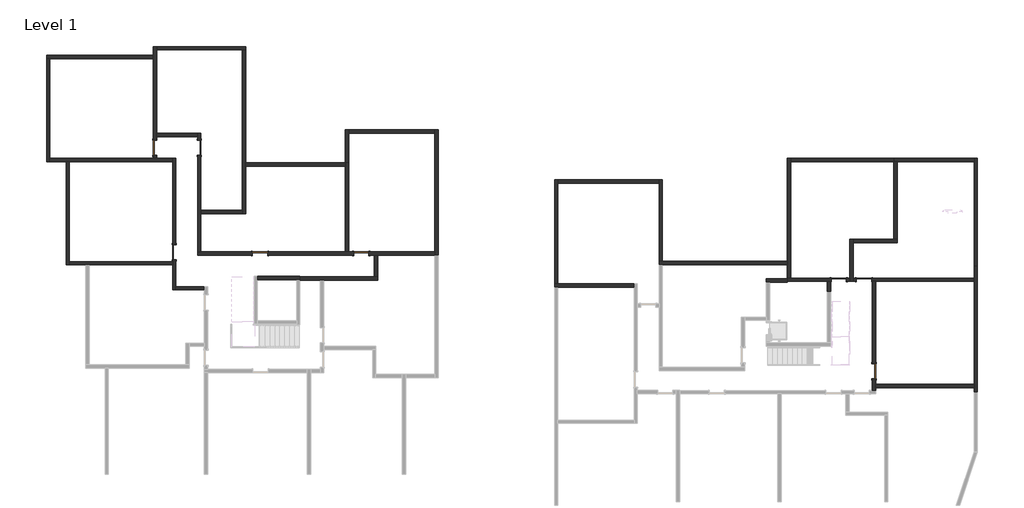
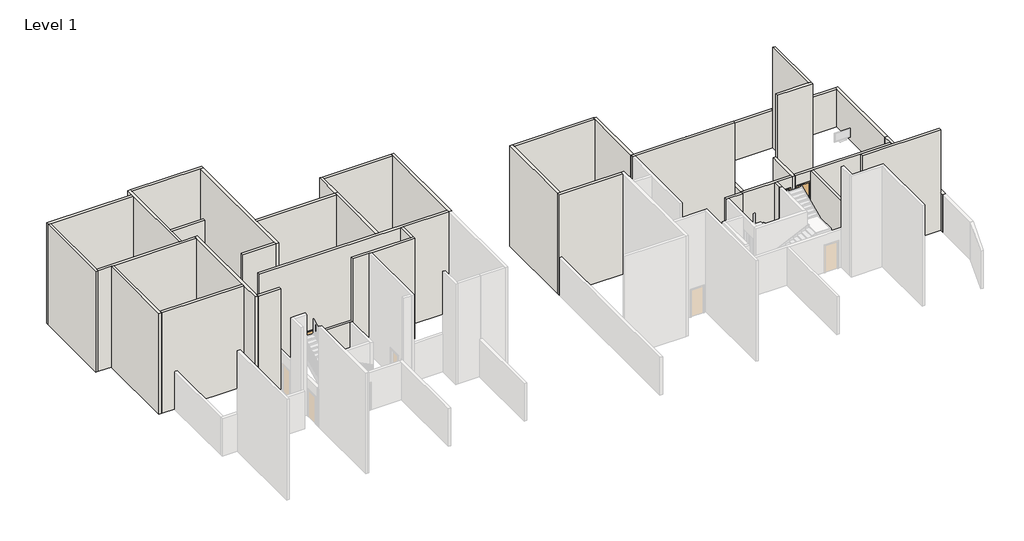
# One storey, part 2 of 3: 41 walls, 8 doors.
"""IFC4 building model written with IfcOpenShell, lengths in millimetres."""

import ifcopenshell
import ifcopenshell.guid

model = None  # the IFC model being written
_history = None  # IfcOwnerHistory: only IFC2X3 demands one
_inside = {}  # id of a spatial element -> (the spatial element, [elements in it])
_under = {}  # id of a project, library or spatial element -> (it, [spatial elements below it])
_declared = {}  # id of a project -> (the project, [libraries it declares])
_typed = {}  # id of a type object -> (the type object, [elements of that type])
_made_of = {}  # id of a material, layer set ... -> (it, [elements and type objects made of it])


def new_model(schema):
    """Start an empty IFC model of exactly this schema.

    Asked for "IFC4X3", IfcOpenShell would pick the latest addendum, in which some entities
    have other attributes; the version numbers below select the first issue.
    IFC2X3 requires an IfcOwnerHistory on every rooted entity: one is made here for all.
    """
    global model, _history
    if schema == "IFC4X3":
        model = ifcopenshell.file(schema_version=(4, 3, 0, 0))
    else:
        model = ifcopenshell.file(schema=schema)
    _inside.clear()
    _under.clear()
    _declared.clear()
    _typed.clear()
    _made_of.clear()
    _history = None
    if model.schema == "IFC2X3":
        org = make("IfcOrganization", Name="unknown")
        user = make(
            "IfcPersonAndOrganization",
            ThePerson=make("IfcPerson", FamilyName="unknown"),
            TheOrganization=org,
        )
        app = make(
            "IfcApplication",
            ApplicationDeveloper=org,
            Version="unknown",
            ApplicationFullName="unknown",
            ApplicationIdentifier="unknown",
        )
        _history = make(
            "IfcOwnerHistory",
            OwningUser=user,
            OwningApplication=app,
            ChangeAction="ADDED",
            CreationDate=0,
        )
    return model


def make(cls, **values):
    """One entity of the class cls with the attributes given. An attribute that is None is left unset."""
    return model.create_entity(
        cls, **{name: value for name, value in values.items() if value is not None}
    )


def rooted(cls, **values):
    """An entity with a GlobalId (a new one), such as an element, a storey or a relation."""
    return make(cls, GlobalId=ifcopenshell.guid.new(), OwnerHistory=_history, **values)


def si_unit(unit_type, name, prefix=None):
    """IfcSIUnit, for example si_unit("LENGTHUNIT", "METRE", prefix="MILLI")."""
    return make("IfcSIUnit", UnitType=unit_type, Prefix=prefix, Name=name)


def assignment(units):
    """IfcUnitAssignment: the units of a project."""
    return None if units is None else make("IfcUnitAssignment", Units=units)


def point(xyz):
    """IfcCartesianPoint."""
    return None if xyz is None else make("IfcCartesianPoint", Coordinates=xyz)


def direction(xyz):
    """IfcDirection."""
    return None if xyz is None else make("IfcDirection", DirectionRatios=xyz)


def frame(location, z_axis=None, x_axis=None):
    """IfcAxis2Placement3D, a coordinate frame: its origin and axes. An axis left out is left unset."""
    return make(
        "IfcAxis2Placement3D",
        Location=point(location),
        Axis=direction(z_axis),
        RefDirection=direction(x_axis),
    )


def origin():
    """The frame at (0, 0, 0) with its axes left unset."""
    return frame((0.0, 0.0, 0.0))


def origin_with_axes():
    """The frame at (0, 0, 0) with the z axis (0, 0, 1) and the x axis (1, 0, 0) written out."""
    return frame((0.0, 0.0, 0.0), z_axis=(0.0, 0.0, 1.0), x_axis=(1.0, 0.0, 0.0))


def place(relative_to, where):
    """IfcLocalPlacement: puts the frame where relative to a parent placement (None: the world)."""
    return make(
        "IfcLocalPlacement", PlacementRelTo=relative_to, RelativePlacement=where
    )


def context(
    kind, dimensions, precision=None, world=None, true_north=None, identifier=None
):
    """IfcGeometricRepresentationContext, for example the 3D "Model" context."""
    return make(
        "IfcGeometricRepresentationContext",
        ContextIdentifier=identifier,
        ContextType=kind,
        CoordinateSpaceDimension=dimensions,
        Precision=precision,
        WorldCoordinateSystem=world,
        TrueNorth=true_north,
    )


def project(units=None, contexts=None):
    """IfcProject with its units and contexts."""
    return rooted(
        "IfcProject",
        Name="project",
        RepresentationContexts=contexts,
        UnitsInContext=assignment(units),
    )


def spatial(cls, under=None, at=None, **own):
    """A site, building, storey or space (cls), placed at a placement, below another one or the project."""
    s = rooted(cls, ObjectPlacement=at, **own)
    if under is not None:
        _under.setdefault(under.id(), (under, []))[1].append(s)
    return s


def polyline(points):
    """IfcPolyline through the points."""
    return make("IfcPolyline", Points=[point(p) for p in points])


def outline(outer, holes=None, kind="AREA"):
    """IfcArbitraryClosedProfileDef: a profile drawn as a closed curve; with holes, ...WithVoids."""
    if holes is None:
        return make("IfcArbitraryClosedProfileDef", ProfileType=kind, OuterCurve=outer)
    return make(
        "IfcArbitraryProfileDefWithVoids",
        ProfileType=kind,
        OuterCurve=outer,
        InnerCurves=holes,
    )


def extrude(swept, where, along, depth):
    """IfcExtrudedAreaSolid: the profile swept, set in the frame where, extruded along a direction by depth."""
    return make(
        "IfcExtrudedAreaSolid",
        SweptArea=swept,
        Position=where,
        ExtrudedDirection=direction(along),
        Depth=depth,
    )


def faces_of(points, faces, orient=None, outer=None):
    """IfcFace entities. A face is a list of loops; a loop is a list of indices into points, from 0.

    orient and outer hold one flag for each loop. By default every Orientation is true, the
    first loop of a face is its IfcFaceOuterBound and the others are IfcFaceBound.
    """
    made = []
    for i, loops in enumerate(faces):
        bounds = []
        for j, loop in enumerate(loops):
            is_outer = j == 0 if outer is None else outer[i][j]
            bounds.append(
                make(
                    "IfcFaceOuterBound" if is_outer else "IfcFaceBound",
                    Bound=make("IfcPolyLoop", Polygon=[points[k] for k in loop]),
                    Orientation=True if orient is None else orient[i][j],
                )
            )
        made.append(make("IfcFace", Bounds=bounds))
    return made


def faceted_brep(points, faces, orient=None, outer=None, voids=None):
    """IfcFacetedBrep: a solid bounded by flat faces; with voids (closed shells), ...WithVoids."""
    shared = [point(p) for p in points]
    hull = make("IfcClosedShell", CfsFaces=faces_of(shared, faces, orient, outer))
    if voids is None:
        return make("IfcFacetedBrep", Outer=hull)
    return make(
        "IfcFacetedBrepWithVoids",
        Outer=hull,
        Voids=[
            make(cls, CfsFaces=faces_of(shared, fs, o, b)) for cls, fs, o, b in voids
        ],
    )


def shape(context_of_items, identifier, shape_type, items):
    """IfcShapeRepresentation: the items that make up one representation, for example the "Body"."""
    return make(
        "IfcShapeRepresentation",
        ContextOfItems=context_of_items,
        RepresentationIdentifier=identifier,
        RepresentationType=shape_type,
        Items=items,
    )


def source(mapping_origin, context_of_items, identifier, shape_type, items):
    """IfcRepresentationMap: a shape defined once, which mapped items show again and again."""
    return make(
        "IfcRepresentationMap",
        MappingOrigin=mapping_origin,
        MappedRepresentation=shape(context_of_items, identifier, shape_type, items),
    )


def transform(
    local_origin,
    x_axis=None,
    y_axis=None,
    z_axis=None,
    scale=None,
    scale2=None,
    scale3=None,
    uniform=True,
):
    """IfcCartesianTransformationOperator3D, or its non-uniform kind. x_axis, y_axis, z_axis: its Axis1, 2, 3."""
    if uniform:
        return make(
            "IfcCartesianTransformationOperator3D",
            Axis1=direction(x_axis),
            Axis2=direction(y_axis),
            LocalOrigin=point(local_origin),
            Scale=scale,
            Axis3=direction(z_axis),
        )
    return make(
        "IfcCartesianTransformationOperator3DnonUniform",
        Axis1=direction(x_axis),
        Axis2=direction(y_axis),
        LocalOrigin=point(local_origin),
        Scale=scale,
        Axis3=direction(z_axis),
        Scale2=scale2,
        Scale3=scale3,
    )


def mapped(mapping_source, mapping_target):
    """IfcMappedItem: shows the shape of a source again, moved by a transform."""
    return make(
        "IfcMappedItem", MappingSource=mapping_source, MappingTarget=mapping_target
    )


def made_of(thing, what):
    """Note that an element or type object is made of a material, layer set ...; save() writes the relation."""
    if what is not None:
        _made_of.setdefault(what.id(), (what, []))[1].append(thing)
    return thing


def element(
    cls,
    number,
    at=None,
    inside=None,
    cuts=None,
    type_object=None,
    material=None,
    context=None,
    identifier="Body",
    shape_type=None,
    held_by="IfcProductDefinitionShape",
    body=None,
    shapes=None,
    **own,
):
    """One element of the class cls, such as IfcWall. Its Tag is "e" and its number.

    at: its placement. inside: the storey or other place that contains it. cuts: it is an
    opening in that element (IfcRelVoidsElement). A single representation is given by context,
    identifier, shape_type and body (its items); several are given by shapes. held_by: the class
    of the entity that holds the representations. save() writes the other relations.
    """
    e = rooted(cls, Tag="e%d" % number, ObjectPlacement=at, **own)
    if body is not None:
        shapes = [shape(context, identifier, shape_type, body)]
    if shapes is not None:
        e.Representation = make(held_by, Representations=shapes)
    if inside is not None:
        _inside.setdefault(inside.id(), (inside, []))[1].append(e)
    if cuts is not None:
        rooted(
            "IfcRelVoidsElement", RelatingBuildingElement=cuts, RelatedOpeningElement=e
        )
    if type_object is not None:
        _typed.setdefault(type_object.id(), (type_object, []))[1].append(e)
    return made_of(e, material)


def aggregate(whole, parts):
    """IfcRelAggregates: a whole, such as a stair, and the parts it consists of."""
    return rooted("IfcRelAggregates", RelatingObject=whole, RelatedObjects=parts)


def save(model, path):
    """Write the relations noted so far, then the file.

    IfcRelAggregates (storeys below a building ...), IfcRelContainedInSpatialStructure (elements
    in a storey), IfcRelDefinesByType, IfcRelAssociatesMaterial and IfcRelDeclares: one each for
    every whole, place, type object, material and project.
    """
    for whole, parts in _under.values():
        aggregate(whole, parts)
    for where, things in _inside.values():
        rooted(
            "IfcRelContainedInSpatialStructure",
            RelatedElements=things,
            RelatingStructure=where,
        )
    for kind, things in _typed.values():
        rooted("IfcRelDefinesByType", RelatedObjects=things, RelatingType=kind)
    for what, things in _made_of.values():
        rooted("IfcRelAssociatesMaterial", RelatedObjects=things, RelatingMaterial=what)
    for by, libraries in _declared.values():
        rooted("IfcRelDeclares", RelatingContext=by, RelatedDefinitions=libraries)
    model.write(path)


def m_single_flush_0915_x_2134mm_727434cd(model_context):
    return source(origin(), model_context, "Body", "SweptSolid", [
        extrude(outline(polyline([(2210.0, -533.5), (0.0, -533.5), (0.0, -457.5), (2134.0, -457.5), (2134.0, 457.5), (0.0, 457.5), (0.0, 533.5), (2210.0, 533.5), (2210.0, -533.5)])), frame((0.0, -125.0, 0.0), z_axis=(0.0, 1.0, 0.0), x_axis=(0.0, 0.0, 1.0)), (0.0, 0.0, 1.0), 25.0),
        extrude(outline(polyline([(2210.0, 533.5), (2210.0, -533.5), (0.0, -533.5), (0.0, -457.5), (2134.0, -457.5), (2134.0, 457.5), (0.0, 457.5), (0.0, 533.5), (2210.0, 533.5)])), frame((0.0, 100.0, 0.0), z_axis=(0.0, 1.0, 0.0), x_axis=(0.0, 0.0, 1.0)), (0.0, 0.0, 1.0), 25.0),
        extrude(outline(polyline([(457.5, -49.0), (457.5, -100.0), (-457.5, -100.0), (-457.5, -49.0), (457.5, -49.0)])), origin_with_axes(), (0.0, 0.0, 1.0), 2134.0),
    ])


def m_single_flush_0915_x_2134mm_6a9e8738(model_context):
    return source(origin(), model_context, "Body", "SweptSolid", [
        extrude(outline(polyline([(2210.0, -533.5), (0.0, -533.5), (0.0, -457.5), (2134.0, -457.5), (2134.0, 457.5), (0.0, 457.5), (0.0, 533.5), (2210.0, 533.5), (2210.0, -533.5)])), frame((0.0, 100.0, 0.0), z_axis=(0.0, 1.0, 0.0), x_axis=(0.0, 0.0, 1.0)), (0.0, 0.0, 1.0), 25.0),
        extrude(outline(polyline([(2210.0, 533.5), (2210.0, -533.5), (0.0, -533.5), (0.0, -457.5), (2134.0, -457.5), (2134.0, 457.5), (0.0, 457.5), (0.0, 533.5), (2210.0, 533.5)])), frame((0.0, -125.0, 0.0), z_axis=(0.0, 1.0, 0.0), x_axis=(0.0, 0.0, 1.0)), (0.0, 0.0, 1.0), 25.0),
        extrude(outline(polyline([(457.5, 49.0), (-457.5, 49.0), (-457.5, 100.0), (457.5, 100.0), (457.5, 49.0)])), origin_with_axes(), (0.0, 0.0, 1.0), 2134.0),
    ])


model = new_model("IFC4")

# Units and contexts
model_context = context("Model", 3, world=origin())
ifc_project = project(units=[si_unit("LENGTHUNIT", "METRE", prefix="MILLI")], contexts=[model_context])

# Site, building, storey
site = spatial("IfcSite", under=ifc_project)
building = spatial("IfcBuilding", under=site)
storey = spatial("IfcBuildingStorey", under=building, Name="Level 1", Elevation=0.0)

# Doors
placement = place(None, origin())
m_single_flush_0915_x_2134mm_shape = m_single_flush_0915_x_2134mm_727434cd(model_context)
element("IfcDoor", 1, ObjectType="M_Single-Flush : 0915 x 2134mm", at=placement, inside=storey, context=model_context, shape_type="MappedRepresentation", body=[
    mapped(m_single_flush_0915_x_2134mm_shape, transform((23447.336337, 519.475628, 0.0), x_axis=(-1.0, 0.0, 0.0), y_axis=(0.0, -1.0, 0.0), z_axis=(0.0, 0.0, 1.0))),
])
element("IfcDoor", 2, ObjectType="M_Single-Flush : 0915 x 2134mm", at=placement, inside=storey, context=model_context, shape_type="MappedRepresentation", body=[
    mapped(m_single_flush_0915_x_2134mm_shape, transform((-6772.8449834, 2100.8372871, 0.0), x_axis=(-1.0, 0.0, 0.0), y_axis=(0.0, -1.0, 0.0), z_axis=(0.0, 0.0, 1.0))),
])
element("IfcDoor", 3, ObjectType="M_Single-Flush : 0915 x 2134mm", at=placement, inside=storey, context=model_context, shape_type="MappedRepresentation", body=[
    mapped(m_single_flush_0915_x_2134mm_shape, transform((-19189.8304233, 8462.8400285, 0.0), x_axis=(0.0, -1.0, 0.0), y_axis=(1.0, 0.0, 0.0), z_axis=(0.0, 0.0, 1.0))),
])
element("IfcDoor", 4, ObjectType="M_Single-Flush : 0915 x 2134mm", at=placement, inside=storey, context=model_context, shape_type="MappedRepresentation", body=[
    mapped(m_single_flush_0915_x_2134mm_shape, transform((-18023.9741722, 2170.3400285, 0.0), x_axis=(0.0, -1.0, 0.0), y_axis=(1.0, 0.0, 0.0), z_axis=(0.0, 0.0, 1.0))),
])
element("IfcDoor", 5, ObjectType="M_Single-Flush : 0915 x 2134mm", at=placement, inside=storey, context=model_context, shape_type="MappedRepresentation", body=[
    mapped(m_single_flush_0915_x_2134mm_shape, transform((-12866.4741722, 2100.8372871, 0.0), x_axis=(-1.0, 0.0, 0.0), y_axis=(0.0, -1.0, 0.0), z_axis=(0.0, 0.0, 1.0))),
])
m_single_flush_0915_x_2134mm_2_shape = m_single_flush_0915_x_2134mm_6a9e8738(model_context)
element("IfcDoor", 6, ObjectType="M_Single-Flush : 0915 x 2134mm", at=placement, inside=storey, context=model_context, shape_type="MappedRepresentation", body=[
    mapped(m_single_flush_0915_x_2134mm_2_shape, transform((24048.8612349, -4982.5098119, 0.0), x_axis=(0.0, -1.0, 0.0), y_axis=(1.0, 0.0, 0.0), z_axis=(0.0, 0.0, 1.0))),
])
element("IfcDoor", 7, ObjectType="M_Single-Flush : 0915 x 2134mm", at=placement, inside=storey, context=model_context, shape_type="MappedRepresentation", body=[
    mapped(m_single_flush_0915_x_2134mm_2_shape, transform((21932.336337, 519.475628, 0.0), x_axis=(1.0, 0.0, 0.0), y_axis=(0.0, 1.0, 0.0), z_axis=(0.0, 0.0, 1.0))),
])
element("IfcDoor", 8, ObjectType="M_Single-Flush : 0915 x 2134mm", at=placement, inside=storey, context=model_context, shape_type="MappedRepresentation", body=[
    mapped(m_single_flush_0915_x_2134mm_2_shape, transform((-16523.9741722, 8455.3400285, 0.0), x_axis=(0.0, -1.0, 0.0), y_axis=(1.0, 0.0, 0.0), z_axis=(0.0, 0.0, 1.0))),
])

# Walls
element("IfcWall", 9, ObjectType="Generic - 200mm", at=placement, inside=storey, context=model_context, shape_type="Brep", body=[
    faceted_brep([(25249.836337, 7619.475628, 0.0), (25449.836337, 7619.475628, 0.0), (30068.3425199, 7619.475628, 0.0), (30068.3425199, 7619.475628, 3000.0), (25249.836337, 7619.475628, 3000.0), (25249.836337, 7819.475628, 0.0), (25249.836337, 7819.475628, 3000.0), (30068.3425199, 7819.475628, 3000.0), (30068.3425199, 7819.475628, 0.0)], [[[0, 1, 2, 3, 4]], [[5, 6, 7, 8]], [[2, 1, 0, 5, 8]], [[4, 3, 7, 6]], [[3, 2, 8, 7]], [[0, 4, 6, 5]]]),
])
element("IfcWall", 10, ObjectType="Generic - 200mm", at=placement, inside=storey, context=model_context, shape_type="Brep", body=[
    faceted_brep([(30068.3425199, 7819.475628, 0.0), (30068.3425199, 7619.475628, 0.0), (30068.3425199, 1319.475628, 0.0), (30068.3425199, 1319.475628, 3000.0), (30068.3425199, 7619.475628, 3000.0), (30068.3425199, 7819.475628, 3000.0), (30268.3425199, 7819.475628, 0.0), (30268.3425199, 7819.475628, 3000.0), (30268.3425199, 1319.475628, 3000.0), (30268.3425199, 1319.475628, 0.0), (30068.8612349, 1319.475628, 0.0), (30068.8612349, 1319.475628, 3000.0)], [[[0, 1, 2, 3, 4, 5]], [[6, 7, 8, 9]], [[2, 1, 0, 6, 9, 10]], [[3, 2, 10, 9, 8, 11]], [[5, 4, 3, 11, 8, 7]], [[0, 5, 7, 6]]]),
])
element("IfcWall", 11, ObjectType="Generic - 200mm", at=placement, inside=storey, context=model_context, shape_type="Brep", body=[
    faceted_brep([(30068.8612349, 1319.475628, 0.0), (30068.8612349, 619.475628, 0.0), (30068.8612349, 419.475628, 0.0), (30068.8612349, -5760.0098119, 0.0), (30068.8612349, -5960.0098119, 0.0), (30068.8612349, -6240.0098119, 0.0), (30068.8612349, -6240.0098119, 3000.0), (30068.8612349, 419.475628, 3000.0), (30068.8612349, 619.475628, 3000.0), (30068.8612349, 1319.475628, 3000.0), (30268.8612349, 1319.475628, 0.0), (30268.8612349, 1319.475628, 3000.0), (30268.8612349, -6240.0098119, 3000.0), (30268.8612349, -6240.0098119, 0.0), (30268.3425199, 1319.475628, 0.0), (30069.3799498, -6240.0098119, 0.0), (30069.3799498, -6240.0098119, 3000.0), (30268.3425199, 1319.475628, 3000.0)], [[[0, 1, 2, 3, 4, 5, 6, 7, 8, 9]], [[10, 11, 12, 13]], [[5, 4, 3, 2, 1, 0, 14, 10, 13, 15]], [[6, 5, 15, 13, 12, 16]], [[9, 8, 7, 6, 16, 12, 11, 17]], [[0, 9, 17, 11, 10, 14]]]),
])
element("IfcWall", 12, ObjectType="Generic - 200mm", at=placement, inside=storey, context=model_context, shape_type="Brep", body=[
    faceted_brep([(24148.8612349, 419.475628, 3000.0), (24148.8612349, -6140.0098119, 3000.0), (24148.8612349, -6140.0098119, 0.0), (24148.8612349, -5960.0098119, 0.0), (24148.8612349, -5760.0098119, 0.0), (24148.8612349, -5440.0098119, 0.0), (24148.8612349, -5440.0098119, 2134.0), (24148.8612349, -4525.0098119, 2134.0), (24148.8612349, -4525.0098119, 0.0), (24148.8612349, 419.475628, 0.0), (23948.8612349, -6140.0098119, 3000.0), (23948.8612349, 419.475628, 3000.0), (23948.8612349, 419.475628, 0.0), (23948.8612349, -4525.0098119, 0.0), (23948.8612349, -4525.0098119, 2134.0), (23948.8612349, -5440.0098119, 2134.0), (23948.8612349, -5440.0098119, 0.0), (23948.8612349, -6140.0098119, 0.0)], [[[0, 1, 2, 3, 4, 5, 6, 7, 8, 9]], [[10, 11, 12, 13, 14, 15, 16, 17]], [[12, 9, 8, 13]], [[2, 17, 16, 5, 4, 3]], [[1, 0, 11, 10]], [[0, 9, 12, 11]], [[15, 6, 5, 16]], [[7, 14, 13, 8]], [[14, 7, 6, 15]], [[2, 1, 10, 17]]]),
])
element("IfcWall", 13, ObjectType="Generic - 200mm", at=placement, inside=storey, context=model_context, shape_type="SweptSolid", body=[
    extrude(outline(polyline([(21449.836337, 419.475628), (21449.836337, -200.524372), (21249.836337, -200.524372), (21249.836337, 419.475628), (21449.836337, 419.475628)])), origin_with_axes(), (0.0, 0.0, 1.0), 3000.0),
])
element("IfcWall", 14, ObjectType="Generic - 200mm", at=placement, inside=storey, context=model_context, shape_type="SweptSolid", body=[
    extrude(outline(polyline([(25249.836337, 7619.475628), (19028.8612349, 7619.475628), (19028.8612349, 7819.475628), (25249.836337, 7819.475628), (25249.836337, 7619.475628)])), origin_with_axes(), (0.0, 0.0, 1.0), 3000.0),
])
element("IfcWall", 15, ObjectType="Generic - 200mm", at=placement, inside=storey, context=model_context, shape_type="Brep", body=[
    faceted_brep([(22789.836337, 419.475628, 0.0), (22789.836337, 619.475628, 0.0), (22789.836337, 2754.475628, 0.0), (22789.836337, 2954.475628, 0.0), (22789.836337, 2954.475628, 3000.0), (22789.836337, 619.475628, 3000.0), (22789.836337, 419.475628, 3000.0), (22589.836337, 419.475628, 0.0), (22589.836337, 419.475628, 3000.0), (22589.836337, 619.475628, 3000.0), (22589.836337, 2954.475628, 3000.0), (22589.836337, 2954.475628, 0.0), (22589.836337, 619.475628, 0.0)], [[[0, 1, 2, 3, 4, 5, 6]], [[7, 8, 9, 10, 11, 12]], [[3, 2, 1, 0, 7, 12, 11]], [[6, 5, 4, 10, 9, 8]], [[0, 6, 8, 7]], [[4, 3, 11, 10]]]),
])
element("IfcWall", 16, ObjectType="Generic - 200mm", at=placement, inside=storey, context=model_context, shape_type="Brep", body=[
    faceted_brep([(18828.8612349, 7819.475628, 0.0), (18828.8612349, 1619.475628, 0.0), (18828.8612349, 1419.475628, 0.0), (18828.8612349, 619.475628, 0.0), (18828.8612349, 619.475628, 3000.0), (18828.8612349, 7819.475628, 3000.0), (19028.8612349, 7819.475628, 0.0), (19028.8612349, 7819.475628, 3000.0), (19028.8612349, 7619.475628, 3000.0), (19028.8612349, 619.475628, 3000.0), (19028.8612349, 619.475628, 0.0), (19028.8612349, 7619.475628, 0.0)], [[[0, 1, 2, 3, 4, 5]], [[6, 7, 8, 9, 10, 11]], [[3, 2, 1, 0, 6, 11, 10]], [[5, 4, 9, 8, 7]], [[4, 3, 10, 9]], [[0, 5, 7, 6]]]),
])
element("IfcWall", 17, ObjectType="Generic - 200mm", at=placement, inside=storey, context=model_context, shape_type="Brep", body=[
    faceted_brep([(30068.8612349, 419.475628, 3000.0), (24148.8612349, 419.475628, 3000.0), (23948.8612349, 419.475628, 3000.0), (22789.836337, 419.475628, 3000.0), (22789.836337, 419.475628, 0.0), (22989.836337, 419.475628, 0.0), (22989.836337, 419.475628, 2134.0), (23904.836337, 419.475628, 2134.0), (23904.836337, 419.475628, 0.0), (23948.8612349, 419.475628, 0.0), (24148.8612349, 419.475628, 0.0), (30068.8612349, 419.475628, 0.0), (22789.836337, 619.475628, 3000.0), (30068.8612349, 619.475628, 3000.0), (30068.8612349, 619.475628, 0.0), (23904.836337, 619.475628, 0.0), (23904.836337, 619.475628, 2134.0), (22989.836337, 619.475628, 2134.0), (22989.836337, 619.475628, 0.0), (22789.836337, 619.475628, 0.0)], [[[0, 1, 2, 3, 4, 5, 6, 7, 8, 9, 10, 11]], [[12, 13, 14, 15, 16, 17, 18, 19]], [[14, 11, 10, 9, 8, 15]], [[4, 19, 18, 5]], [[3, 2, 1, 0, 13, 12]], [[0, 11, 14, 13]], [[4, 3, 12, 19]], [[17, 6, 5, 18]], [[7, 16, 15, 8]], [[16, 7, 6, 17]]]),
])
element("IfcWall", 18, ObjectType="Generic - 200mm", at=placement, inside=storey, context=model_context, shape_type="Brep", body=[
    faceted_brep([(18828.8612349, 579.475628, 0.0), (17570.6041014, 579.475628, 0.0), (17570.6041014, 579.475628, 3000.0), (18828.8612349, 579.475628, 3000.0), (18828.8612349, 379.475628, 0.0), (18828.8612349, 379.475628, 3000.0), (17770.6041014, 379.475628, 3000.0), (17570.6041014, 379.475628, 3000.0), (17570.6041014, 379.475628, 0.0), (17770.6041014, 379.475628, 0.0), (18828.8612349, 419.475628, 0.0), (18828.8612349, 419.475628, 3000.0)], [[[0, 1, 2, 3]], [[4, 5, 6, 7, 8, 9]], [[1, 0, 10, 4, 9, 8]], [[2, 1, 8, 7]], [[3, 2, 7, 6, 5, 11]], [[0, 3, 11, 5, 4, 10]]]),
])
element("IfcWall", 19, ObjectType="Generic - 200mm", at=placement, inside=storey, context=model_context, shape_type="Brep", body=[
    faceted_brep([(18828.8612349, 619.475628, 3000.0), (19028.8612349, 619.475628, 3000.0), (22589.836337, 619.475628, 3000.0), (22589.836337, 619.475628, 0.0), (22389.836337, 619.475628, 0.0), (22389.836337, 619.475628, 2134.0), (21474.836337, 619.475628, 2134.0), (21474.836337, 619.475628, 0.0), (19028.8612349, 619.475628, 0.0), (18828.8612349, 619.475628, 0.0), (22589.836337, 419.475628, 3000.0), (21449.836337, 419.475628, 3000.0), (21249.836337, 419.475628, 3000.0), (18828.8612349, 419.475628, 3000.0), (18828.8612349, 419.475628, 0.0), (21249.836337, 419.475628, 0.0), (21449.836337, 419.475628, 0.0), (21474.836337, 419.475628, 0.0), (21474.836337, 419.475628, 2134.0), (22389.836337, 419.475628, 2134.0), (22389.836337, 419.475628, 0.0), (22589.836337, 419.475628, 0.0), (18828.8612349, 579.475628, 0.0), (18828.8612349, 579.475628, 3000.0)], [[[0, 1, 2, 3, 4, 5, 6, 7, 8, 9]], [[10, 11, 12, 13, 14, 15, 16, 17, 18, 19, 20, 21]], [[3, 21, 20, 4]], [[14, 22, 9, 8, 7, 17, 16, 15]], [[2, 1, 0, 23, 13, 12, 11, 10]], [[0, 9, 22, 14, 13, 23]], [[3, 2, 10, 21]], [[19, 5, 4, 20]], [[6, 18, 17, 7]], [[18, 6, 5, 19]]]),
])
element("IfcWall", 20, ObjectType="Generic - 200mm", at=placement, inside=storey, context=model_context, shape_type="Brep", body=[
    faceted_brep([(22789.836337, 2754.475628, 0.0), (25449.836337, 2754.475628, 0.0), (25449.836337, 2754.475628, 8000.0), (22789.836337, 2754.475628, 8000.0), (22789.836337, 2954.475628, 0.0), (22789.836337, 2954.475628, 3000.0), (22789.836337, 2954.475628, 8000.0), (25249.836337, 2954.475628, 8000.0), (25449.836337, 2954.475628, 8000.0), (25449.836337, 2954.475628, 0.0), (25249.836337, 2954.475628, 0.0)], [[[0, 1, 2, 3]], [[4, 5, 6, 7, 8, 9, 10]], [[1, 0, 4, 10, 9]], [[3, 2, 8, 7, 6]], [[2, 1, 9, 8]], [[0, 3, 6, 5, 4]]]),
])
element("IfcWall", 21, ObjectType="Generic - 200mm", at=placement, inside=storey, context=model_context, shape_type="Brep", body=[
    faceted_brep([(25449.836337, 2954.475628, 0.0), (25449.836337, 7619.475628, 0.0), (25449.836337, 7619.475628, 8000.0), (25449.836337, 2954.475628, 8000.0), (25249.836337, 2954.475628, 0.0), (25249.836337, 2954.475628, 8000.0), (25249.836337, 7619.475628, 8000.0), (25249.836337, 7619.475628, 3000.0), (25249.836337, 7619.475628, 0.0)], [[[0, 1, 2, 3]], [[4, 5, 6, 7, 8]], [[1, 0, 4, 8]], [[3, 2, 6, 5]], [[0, 3, 5, 4]], [[2, 1, 8, 7, 6]]]),
])
element("IfcWall", 22, ObjectType="Generic - 200mm", at=placement, inside=storey, context=model_context, shape_type="SweptSolid", body=[
    extrude(outline(polyline([(30068.8612349, -5960.0098119), (24148.8612349, -5960.0098119), (24148.8612349, -5760.0098119), (30068.8612349, -5760.0098119), (30068.8612349, -5960.0098119)])), origin_with_axes(), (0.0, 0.0, 1.0), 8000.0),
])
element("IfcWall", 23, ObjectType="Generic - 200mm", at=placement, inside=storey, context=model_context, shape_type="Brep", body=[
    faceted_brep([(-10469.8304233, 720.8372871, 0.0), (-13026.101437, 720.8372871, 0.0), (-13026.101437, 720.8372871, 3000.0), (-10469.8304233, 720.8372871, 3000.0), (-10469.8304233, 520.8372871, 0.0), (-10469.8304233, 520.8372871, 3000.0), (-10669.8304233, 520.8372871, 3000.0), (-13026.101437, 520.8372871, 3000.0), (-13026.101437, 520.8372871, 0.0), (-10669.8304233, 520.8372871, 0.0), (-10469.8304233, 700.8372871, 0.0)], [[[0, 1, 2, 3]], [[4, 5, 6, 7, 8, 9]], [[1, 0, 10, 4, 9, 8]], [[3, 2, 7, 6, 5]], [[2, 1, 8, 7]], [[0, 3, 5, 4, 10]]]),
])
element("IfcWall", 24, ObjectType="Generic - 200mm", at=placement, inside=storey, context=model_context, shape_type="Brep", body=[
    faceted_brep([(-19089.8304233, 7812.8400285, 0.0), (-19089.8304233, 8005.3400285, 0.0), (-19089.8304233, 8005.3400285, 2134.0), (-19089.8304233, 8920.3400285, 2134.0), (-19089.8304233, 8920.3400285, 0.0), (-19089.8304233, 9112.8400285, 0.0), (-19089.8304233, 9312.8400285, 0.0), (-19089.8304233, 14340.8372871, 0.0), (-19089.8304233, 14540.8372871, 0.0), (-19089.8304233, 14540.8372871, 8000.0), (-19089.8304233, 14340.8372871, 8000.0), (-19089.8304233, 9312.8400285, 8000.0), (-19089.8304233, 9112.8400285, 8000.0), (-19089.8304233, 7812.8400285, 8000.0), (-19289.8304233, 8005.3400285, 2134.0), (-19289.8304233, 8005.3400285, 0.0), (-19289.8304233, 7812.8400285, 0.0), (-19289.8304233, 7812.8400285, 8000.0), (-19289.8304233, 13812.8400285, 8000.0), (-19289.8304233, 14012.8400285, 8000.0), (-19289.8304233, 14540.8372871, 8000.0), (-19289.8304233, 14540.8372871, 0.0), (-19289.8304233, 14012.8400285, 0.0), (-19289.8304233, 13812.8400285, 0.0), (-19289.8304233, 8920.3400285, 0.0), (-19289.8304233, 8920.3400285, 2134.0)], [[[0, 1, 2, 3, 4, 5, 6, 7, 8, 9, 10, 11, 12, 13]], [[14, 15, 16, 17, 18, 19, 20, 21, 22, 23, 24, 25]], [[16, 15, 1, 0]], [[24, 23, 22, 21, 8, 7, 6, 5, 4]], [[13, 12, 11, 10, 9, 20, 19, 18, 17]], [[9, 8, 21, 20]], [[0, 13, 17, 16]], [[2, 1, 15, 14]], [[3, 2, 14, 25]], [[4, 3, 25, 24]]]),
])
element("IfcWall", 25, ObjectType="Generic - 200mm", at=placement, inside=storey, context=model_context, shape_type="Brep", body=[
    faceted_brep([(9628.8612349, 279.9901881, 0.0), (5043.716007, 279.9901881, 0.0), (4843.716007, 279.9901881, 0.0), (4843.716007, 279.9901881, 8000.0), (5043.716007, 279.9901881, 8000.0), (9628.8612349, 279.9901881, 8000.0), (9628.8612349, 79.9901881, 0.0), (9628.8612349, 79.9901881, 8000.0), (4843.716007, 79.9901881, 8000.0), (4843.716007, 79.9901881, 3000.0), (4843.716007, 79.9901881, 0.0), (5043.716007, 79.9901881, 0.0)], [[[0, 1, 2, 3, 4, 5]], [[6, 7, 8, 9, 10, 11]], [[2, 1, 0, 6, 11, 10]], [[5, 4, 3, 8, 7]], [[0, 5, 7, 6]], [[2, 10, 9, 8, 3]]]),
])
element("IfcWall", 26, ObjectType="Generic - 200mm", at=placement, inside=storey, context=model_context, shape_type="Brep", body=[
    faceted_brep([(-13726.101437, 14540.8372871, 0.0), (-19089.8304233, 14540.8372871, 0.0), (-19089.8304233, 14540.8372871, 8000.0), (-13726.101437, 14540.8372871, 8000.0), (-13726.101437, 14340.8372871, 0.0), (-13726.101437, 14340.8372871, 8000.0), (-13926.101437, 14340.8372871, 8000.0), (-19089.8304233, 14340.8372871, 8000.0), (-19089.8304233, 14340.8372871, 0.0), (-13926.101437, 14340.8372871, 0.0)], [[[0, 1, 2, 3]], [[4, 5, 6, 7, 8, 9]], [[1, 0, 4, 9, 8]], [[3, 2, 7, 6, 5]], [[2, 1, 8, 7]], [[0, 3, 5, 4]]]),
])
element("IfcWall", 27, ObjectType="Generic - 200mm", at=placement, inside=storey, context=model_context, shape_type="Brep", body=[
    faceted_brep([(-25701.4369496, 13812.8400285, 0.0), (-25701.4369496, 7612.8400285, 0.0), (-25701.4369496, 7612.8400285, 8000.0), (-25701.4369496, 13812.8400285, 8000.0), (-25501.4369496, 13812.8400285, 0.0), (-25501.4369496, 13812.8400285, 8000.0), (-25501.4369496, 7812.8400285, 8000.0), (-25501.4369496, 7612.8400285, 8000.0), (-25501.4369496, 7612.8400285, 0.0), (-25501.4369496, 7812.8400285, 0.0)], [[[0, 1, 2, 3]], [[4, 5, 6, 7, 8, 9]], [[1, 0, 4, 9, 8]], [[3, 2, 7, 6, 5]], [[2, 1, 8, 7]], [[0, 3, 5, 4]]]),
])
element("IfcWall", 28, ObjectType="Generic - 200mm", at=placement, inside=storey, context=model_context, shape_type="Brep", body=[
    faceted_brep([(-25501.4369496, 7612.8400285, 0.0), (-24523.9741722, 7612.8400285, 0.0), (-24323.9741722, 7612.8400285, 0.0), (-18123.9741722, 7612.8400285, 0.0), (-18123.9741722, 7612.8400285, 8000.0), (-24323.9741722, 7612.8400285, 8000.0), (-24523.9741722, 7612.8400285, 8000.0), (-25501.4369496, 7612.8400285, 8000.0), (-25501.4369496, 7812.8400285, 0.0), (-25501.4369496, 7812.8400285, 8000.0), (-19289.8304233, 7812.8400285, 8000.0), (-19089.8304233, 7812.8400285, 8000.0), (-18123.9741722, 7812.8400285, 8000.0), (-18123.9741722, 7812.8400285, 0.0), (-19089.8304233, 7812.8400285, 0.0), (-19289.8304233, 7812.8400285, 0.0)], [[[0, 1, 2, 3, 4, 5, 6, 7]], [[8, 9, 10, 11, 12, 13, 14, 15]], [[3, 2, 1, 0, 8, 15, 14, 13]], [[7, 6, 5, 4, 12, 11, 10, 9]], [[0, 7, 9, 8]], [[4, 3, 13, 12]]]),
])
element("IfcWall", 29, ObjectType="Generic - 200mm", at=placement, inside=storey, context=model_context, shape_type="Brep", body=[
    faceted_brep([(-19289.8304233, 14012.8400285, 0.0), (-25701.4369496, 14012.8400285, 0.0), (-25701.4369496, 14012.8400285, 8000.0), (-19289.8304233, 14012.8400285, 8000.0), (-19289.8304233, 13812.8400285, 0.0), (-19289.8304233, 13812.8400285, 8000.0), (-25501.4369496, 13812.8400285, 8000.0), (-25701.4369496, 13812.8400285, 8000.0), (-25701.4369496, 13812.8400285, 0.0), (-25501.4369496, 13812.8400285, 0.0)], [[[0, 1, 2, 3]], [[4, 5, 6, 7, 8, 9]], [[1, 0, 4, 9, 8]], [[3, 2, 7, 6, 5]], [[2, 1, 8, 7]], [[0, 3, 5, 4]]]),
])
element("IfcWall", 30, ObjectType="Generic - 200mm", at=placement, inside=storey, context=model_context, shape_type="Brep", body=[
    faceted_brep([(-24523.9741722, 7612.8400285, 0.0), (-24523.9741722, 1412.8400285, 0.0), (-24523.9741722, 1412.8400285, 8000.0), (-24523.9741722, 7612.8400285, 8000.0), (-24323.9741722, 7612.8400285, 0.0), (-24323.9741722, 7612.8400285, 8000.0), (-24323.9741722, 1612.8400285, 8000.0), (-24323.9741722, 1412.8400285, 8000.0), (-24323.9741722, 1412.8400285, 0.0), (-24323.9741722, 1612.8400285, 0.0)], [[[0, 1, 2, 3]], [[4, 5, 6, 7, 8, 9]], [[1, 0, 4, 9, 8]], [[3, 2, 7, 6, 5]], [[0, 3, 5, 4]], [[2, 1, 8, 7]]]),
])
element("IfcWall", 31, ObjectType="Generic - 200mm", at=placement, inside=storey, context=model_context, shape_type="Brep", body=[
    faceted_brep([(-24323.9741722, 1412.8400285, 0.0), (-23346.5113948, 1412.8400285, 0.0), (-23146.5113948, 1412.8400285, 0.0), (-18123.9741722, 1412.8400285, 0.0), (-18123.9741722, 1412.8400285, 8000.0), (-24323.9741722, 1412.8400285, 8000.0), (-24323.9741722, 1612.8400285, 0.0), (-24323.9741722, 1612.8400285, 8000.0), (-18123.9741722, 1612.8400285, 8000.0), (-18123.9741722, 1612.8400285, 0.0)], [[[0, 1, 2, 3, 4, 5]], [[6, 7, 8, 9]], [[3, 2, 1, 0, 6, 9]], [[5, 4, 8, 7]], [[0, 5, 7, 6]], [[4, 3, 9, 8]]]),
])
element("IfcWall", 32, ObjectType="Generic - 200mm", at=placement, inside=storey, context=model_context, shape_type="Brep", body=[
    faceted_brep([(-19089.8304233, 9112.8400285, 0.0), (-16623.9741722, 9112.8400285, 0.0), (-16623.9741722, 9112.8400285, 8000.0), (-19089.8304233, 9112.8400285, 8000.0), (-19089.8304233, 9312.8400285, 0.0), (-19089.8304233, 9312.8400285, 8000.0), (-16623.9741722, 9312.8400285, 8000.0), (-16623.9741722, 9312.8400285, 3000.0), (-16623.9741722, 9312.8400285, 0.0)], [[[0, 1, 2, 3]], [[4, 5, 6, 7, 8]], [[1, 0, 4, 8]], [[3, 2, 6, 5]], [[0, 3, 5, 4]], [[2, 1, 8, 7, 6]]]),
])
element("IfcWall", 33, ObjectType="Generic - 200mm", at=placement, inside=storey, context=model_context, shape_type="Brep", body=[
    faceted_brep([(-18123.9741722, 1712.8400285, 2134.0), (-18123.9741722, 1712.8400285, 0.0), (-18123.9741722, 1612.8400285, 0.0), (-18123.9741722, 1412.8400285, 0.0), (-18123.9741722, -87.1599715, 0.0), (-18123.9741722, -87.1599715, 8000.0), (-18123.9741722, 1412.8400285, 8000.0), (-18123.9741722, 1612.8400285, 8000.0), (-18123.9741722, 7612.8400285, 8000.0), (-18123.9741722, 7812.8400285, 8000.0), (-18123.9741722, 7812.8400285, 0.0), (-18123.9741722, 7612.8400285, 0.0), (-18123.9741722, 2627.8400285, 0.0), (-18123.9741722, 2627.8400285, 2134.0), (-17923.9741722, -87.1599715, 0.0), (-17923.9741722, 112.8400285, 0.0), (-17923.9741722, 1712.8400285, 0.0), (-17923.9741722, 1712.8400285, 2134.0), (-17923.9741722, 2627.8400285, 2134.0), (-17923.9741722, 2627.8400285, 0.0), (-17923.9741722, 7812.8400285, 0.0), (-17923.9741722, 7812.8400285, 8000.0), (-17923.9741722, 112.8400285, 8000.0), (-17923.9741722, -87.1599715, 8000.0)], [[[0, 1, 2, 3, 4, 5, 6, 7, 8, 9, 10, 11, 12, 13]], [[14, 15, 16, 17, 18, 19, 20, 21, 22, 23]], [[12, 11, 10, 20, 19]], [[4, 3, 2, 1, 16, 15, 14]], [[9, 8, 7, 6, 5, 23, 22, 21]], [[10, 9, 21, 20]], [[5, 4, 14, 23]], [[17, 16, 1, 0]], [[18, 17, 0, 13]], [[19, 18, 13, 12]]]),
])
element("IfcWall", 34, ObjectType="Generic - 200mm", at=placement, inside=storey, context=model_context, shape_type="Brep", body=[
    faceted_brep([(-7730.3449834, 7540.8372871, 0.0), (-7730.3449834, 7340.8372871, 0.0), (-7730.3449834, 2200.8372871, 0.0), (-7730.3449834, 2200.8372871, 8000.0), (-7730.3449834, 7340.8372871, 8000.0), (-7730.3449834, 7540.8372871, 8000.0), (-7530.3449834, 7540.8372871, 0.0), (-7530.3449834, 7540.8372871, 8000.0), (-7530.3449834, 2200.8372871, 8000.0), (-7530.3449834, 2200.8372871, 0.0)], [[[0, 1, 2, 3, 4, 5]], [[6, 7, 8, 9]], [[2, 1, 0, 6, 9]], [[5, 4, 3, 8, 7]], [[0, 5, 7, 6]], [[3, 2, 9, 8]]]),
])
element("IfcWall", 35, ObjectType="Generic - 200mm", at=placement, inside=storey, context=model_context, shape_type="Brep", body=[
    faceted_brep([(-17923.9741722, -87.1599715, 0.0), (-16213.9741722, -87.1599715, 0.0), (-16213.9741722, -87.1599715, 8000.0), (-17923.9741722, -87.1599715, 8000.0), (-17923.9741722, 112.8400285, 0.0), (-17923.9741722, 112.8400285, 8000.0), (-16213.9741722, 112.8400285, 8000.0), (-16213.9741722, 112.8400285, 3000.0), (-16213.9741722, 112.8400285, 0.0)], [[[0, 1, 2, 3]], [[4, 5, 6, 7, 8]], [[1, 0, 4, 8]], [[3, 2, 6, 5]], [[0, 3, 5, 4]], [[2, 1, 8, 7, 6]]]),
])
element("IfcWall", 36, ObjectType="Generic - 200mm", at=placement, inside=storey, context=model_context, shape_type="Brep", body=[
    faceted_brep([(-16423.9741722, 2200.8372871, 0.0), (-16423.9741722, 4500.8372871, 0.0), (-16423.9741722, 4700.8372871, 0.0), (-16423.9741722, 7997.8400285, 0.0), (-16423.9741722, 7997.8400285, 2134.0), (-16423.9741722, 8912.8400285, 2134.0), (-16423.9741722, 8912.8400285, 0.0), (-16423.9741722, 9312.8400285, 0.0), (-16423.9741722, 9312.8400285, 3000.0), (-16423.9741722, 2200.8372871, 3000.0), (-16623.9741722, 7997.8400285, 2134.0), (-16623.9741722, 7997.8400285, 0.0), (-16623.9741722, 2200.8372871, 0.0), (-16623.9741722, 2200.8372871, 3000.0), (-16623.9741722, 9312.8400285, 3000.0), (-16623.9741722, 9312.8400285, 0.0), (-16623.9741722, 9112.8400285, 0.0), (-16623.9741722, 8912.8400285, 0.0), (-16623.9741722, 8912.8400285, 2134.0)], [[[0, 1, 2, 3, 4, 5, 6, 7, 8, 9]], [[10, 11, 12, 13, 14, 15, 16, 17, 18]], [[12, 11, 3, 2, 1, 0]], [[17, 16, 15, 7, 6]], [[9, 8, 14, 13]], [[0, 9, 13, 12]], [[8, 7, 15, 14]], [[4, 3, 11, 10]], [[5, 4, 10, 18]], [[6, 5, 18, 17]]]),
])
element("IfcWall", 37, ObjectType="Generic - 200mm", at=placement, inside=storey, context=model_context, shape_type="SweptSolid", body=[
    extrude(outline(polyline([(-13726.101437, 7540.8372871), (-7730.3449834, 7540.8372871), (-7730.3449834, 7340.8372871), (-13726.101437, 7340.8372871), (-13726.101437, 7540.8372871)])), origin_with_axes(), (0.0, 0.0, 1.0), 8000.0),
])
element("IfcWall", 38, ObjectType="Generic - 200mm", at=placement, inside=storey, context=model_context, shape_type="Brep", body=[
    faceted_brep([(-16623.9741722, 2000.8372871, 0.0), (-13323.9741722, 2000.8372871, 0.0), (-13323.9741722, 2000.8372871, 2134.0), (-12408.9741722, 2000.8372871, 2134.0), (-12408.9741722, 2000.8372871, 0.0), (-7230.3449834, 2000.8372871, 0.0), (-7230.3449834, 2000.8372871, 2134.0), (-6315.3449834, 2000.8372871, 2134.0), (-6315.3449834, 2000.8372871, 0.0), (-5990.3449834, 2000.8372871, 0.0), (-5790.3449834, 2000.8372871, 0.0), (-2360.3449834, 2000.8372871, 0.0), (-2350.3449834, 2000.8372871, 0.0), (-2350.3449834, 2000.8372871, 8000.0), (-2360.3449834, 2000.8372871, 8000.0), (-5790.3449834, 2000.8372871, 8000.0), (-5990.3449834, 2000.8372871, 8000.0), (-16623.9741722, 2000.8372871, 8000.0), (-13323.9741722, 2200.8372871, 2134.0), (-13323.9741722, 2200.8372871, 0.0), (-16423.9741722, 2200.8372871, 0.0), (-16623.9741722, 2200.8372871, 0.0), (-16623.9741722, 2200.8372871, 3000.0), (-16623.9741722, 2200.8372871, 8000.0), (-7730.3449834, 2200.8372871, 8000.0), (-7530.3449834, 2200.8372871, 8000.0), (-2350.3449834, 2200.8372871, 8000.0), (-2350.3449834, 2200.8372871, 0.0), (-6315.3449834, 2200.8372871, 0.0), (-6315.3449834, 2200.8372871, 2134.0), (-7230.3449834, 2200.8372871, 2134.0), (-7230.3449834, 2200.8372871, 0.0), (-7530.3449834, 2200.8372871, 0.0), (-7730.3449834, 2200.8372871, 0.0), (-12408.9741722, 2200.8372871, 0.0), (-12408.9741722, 2200.8372871, 2134.0)], [[[0, 1, 2, 3, 4, 5, 6, 7, 8, 9, 10, 11, 12, 13, 14, 15, 16, 17]], [[18, 19, 20, 21, 22, 23, 24, 25, 26, 27, 28, 29, 30, 31, 32, 33, 34, 35]], [[28, 27, 12, 11, 10, 9, 8]], [[21, 20, 19, 1, 0]], [[34, 33, 32, 31, 5, 4]], [[17, 16, 15, 14, 13, 26, 25, 24, 23]], [[0, 17, 23, 22, 21]], [[13, 12, 27, 26]], [[6, 5, 31, 30]], [[7, 6, 30, 29]], [[8, 7, 29, 28]], [[2, 1, 19, 18]], [[3, 2, 18, 35]], [[4, 3, 35, 34]]]),
])
element("IfcWall", 39, ObjectType="Generic - 200mm", at=placement, inside=storey, context=model_context, shape_type="Brep", body=[
    faceted_brep([(-5790.3449834, 700.8372871, 0.0), (-5990.3449834, 700.8372871, 0.0), (-10469.8304233, 700.8372871, 0.0), (-10469.8304233, 700.8372871, 8000.0), (-5990.3449834, 700.8372871, 8000.0), (-5790.3449834, 700.8372871, 8000.0), (-5790.3449834, 500.8372871, 0.0), (-5790.3449834, 500.8372871, 8000.0), (-9030.3629108, 500.8372871, 8000.0), (-9230.3629108, 500.8372871, 8000.0), (-10469.8304233, 500.8372871, 8000.0), (-10469.8304233, 500.8372871, 0.0), (-9230.3629108, 500.8372871, 0.0), (-9030.3629108, 500.8372871, 0.0), (-10469.8304233, 520.8372871, 0.0)], [[[0, 1, 2, 3, 4, 5]], [[6, 7, 8, 9, 10, 11, 12, 13]], [[2, 1, 0, 6, 13, 12, 11, 14]], [[5, 4, 3, 10, 9, 8, 7]], [[3, 2, 14, 11, 10]], [[0, 5, 7, 6]]]),
])
element("IfcWall", 40, ObjectType="Generic - 200mm", at=placement, inside=storey, context=model_context, shape_type="Brep", body=[
    faceted_brep([(-2350.3449834, 9540.8372871, 0.0), (-2350.3449834, 9340.8372871, 0.0), (-2350.3449834, 2200.8372871, 0.0), (-2350.3449834, 2000.8372871, 0.0), (-2350.3449834, 2000.8372871, 8000.0), (-2350.3449834, 2200.8372871, 8000.0), (-2350.3449834, 9340.8372871, 8000.0), (-2350.3449834, 9540.8372871, 8000.0), (-2150.3449834, 9540.8372871, 0.0), (-2150.3449834, 9540.8372871, 8000.0), (-2150.3449834, 2000.8372871, 8000.0), (-2150.3449834, 2000.8372871, 0.0), (-2160.3449834, 2000.8372871, 0.0), (-2160.3449834, 2000.8372871, 8000.0)], [[[0, 1, 2, 3, 4, 5, 6, 7]], [[8, 9, 10, 11]], [[3, 2, 1, 0, 8, 11, 12]], [[7, 6, 5, 4, 13, 10, 9]], [[0, 7, 9, 8]], [[4, 3, 12, 11, 10, 13]]]),
])
element("IfcWall", 41, ObjectType="Generic - 200mm", at=placement, inside=storey, context=model_context, shape_type="Brep", body=[
    faceted_brep([(11128.8612349, 1419.475628, 0.0), (11328.8612349, 1419.475628, 0.0), (18828.8612349, 1419.475628, 0.0), (18828.8612349, 1419.475628, 8000.0), (11328.8612349, 1419.475628, 8000.0), (11128.8612349, 1419.475628, 8000.0), (11128.8612349, 1619.475628, 0.0), (11128.8612349, 1619.475628, 8000.0), (11328.8612349, 1619.475628, 8000.0), (18828.8612349, 1619.475628, 8000.0), (18828.8612349, 1619.475628, 0.0), (11328.8612349, 1619.475628, 0.0)], [[[0, 1, 2, 3, 4, 5]], [[6, 7, 8, 9, 10, 11]], [[2, 1, 0, 6, 11, 10]], [[5, 4, 3, 9, 8, 7]], [[3, 2, 10, 9]], [[0, 5, 7, 6]]]),
])
element("IfcWall", 42, ObjectType="Generic - 200mm", at=placement, inside=storey, context=model_context, shape_type="Brep", body=[
    faceted_brep([(5043.716007, 279.9901881, 0.0), (5043.716007, 6319.475628, 0.0), (5043.716007, 6519.475628, 0.0), (5043.716007, 6519.475628, 8000.0), (5043.716007, 6319.475628, 8000.0), (5043.716007, 279.9901881, 8000.0), (4843.716007, 279.9901881, 0.0), (4843.716007, 279.9901881, 8000.0), (4843.716007, 6519.475628, 8000.0), (4843.716007, 6519.475628, 0.0)], [[[0, 1, 2, 3, 4, 5]], [[6, 7, 8, 9]], [[2, 1, 0, 6, 9]], [[5, 4, 3, 8, 7]], [[0, 5, 7, 6]], [[3, 2, 9, 8]]]),
])
element("IfcWall", 43, ObjectType="Generic - 200mm", at=placement, inside=storey, context=model_context, shape_type="Brep", body=[
    faceted_brep([(11328.8612349, 1619.475628, 0.0), (11328.8612349, 6519.475628, 0.0), (11328.8612349, 6519.475628, 8000.0), (11328.8612349, 1619.475628, 8000.0), (11128.8612349, 1619.475628, 0.0), (11128.8612349, 1619.475628, 8000.0), (11128.8612349, 6319.475628, 8000.0), (11128.8612349, 6519.475628, 8000.0), (11128.8612349, 6519.475628, 0.0), (11128.8612349, 6319.475628, 0.0)], [[[0, 1, 2, 3]], [[4, 5, 6, 7, 8, 9]], [[1, 0, 4, 9, 8]], [[3, 2, 7, 6, 5]], [[0, 3, 5, 4]], [[2, 1, 8, 7]]]),
])
element("IfcWall", 44, ObjectType="Generic - 200mm", at=placement, inside=storey, context=model_context, shape_type="SweptSolid", body=[
    extrude(outline(polyline([(5043.716007, 6519.475628), (11128.8612349, 6519.475628), (11128.8612349, 6319.475628), (5043.716007, 6319.475628), (5043.716007, 6519.475628)])), origin_with_axes(), (0.0, 0.0, 1.0), 8000.0),
])
element("IfcWall", 45, ObjectType="Generic - 200mm", at=placement, inside=storey, context=model_context, shape_type="Brep", body=[
    faceted_brep([(-13926.101437, 14340.8372871, 0.0), (-13926.101437, 4700.8372871, 0.0), (-13926.101437, 4500.8372871, 0.0), (-13926.101437, 4500.8372871, 8000.0), (-13926.101437, 4700.8372871, 8000.0), (-13926.101437, 14340.8372871, 8000.0), (-13726.101437, 14340.8372871, 0.0), (-13726.101437, 14340.8372871, 8000.0), (-13726.101437, 7540.8372871, 8000.0), (-13726.101437, 7340.8372871, 8000.0), (-13726.101437, 4500.8372871, 8000.0), (-13726.101437, 4500.8372871, 0.0), (-13726.101437, 7340.8372871, 0.0), (-13726.101437, 7540.8372871, 0.0)], [[[0, 1, 2, 3, 4, 5]], [[6, 7, 8, 9, 10, 11, 12, 13]], [[2, 1, 0, 6, 13, 12, 11]], [[5, 4, 3, 10, 9, 8, 7]], [[3, 2, 11, 10]], [[0, 5, 7, 6]]]),
])
element("IfcWall", 46, ObjectType="Generic - 200mm", at=placement, inside=storey, context=model_context, shape_type="SweptSolid", body=[
    extrude(outline(polyline([(-16423.9741722, 4700.8372871), (-13926.101437, 4700.8372871), (-13926.101437, 4500.8372871), (-16423.9741722, 4500.8372871), (-16423.9741722, 4700.8372871)])), origin_with_axes(), (0.0, 0.0, 1.0), 8000.0),
])
element("IfcWall", 47, ObjectType="Generic - 200mm", at=placement, inside=storey, context=model_context, shape_type="SweptSolid", body=[
    extrude(outline(polyline([(-5790.3449834, 2000.8372871), (-5790.3449834, 700.8372871), (-5990.3449834, 700.8372871), (-5990.3449834, 2000.8372871), (-5790.3449834, 2000.8372871)])), origin_with_axes(), (0.0, 0.0, 1.0), 8000.0),
])
element("IfcWall", 48, ObjectType="Generic - 200mm", at=placement, inside=storey, context=model_context, shape_type="Brep", body=[
    faceted_brep([(-7530.3449834, 7540.8372871, 0.0), (-7530.3449834, 9340.8372871, 0.0), (-7530.3449834, 9540.8372871, 0.0), (-7530.3449834, 9540.8372871, 8000.0), (-7530.3449834, 9340.8372871, 8000.0), (-7530.3449834, 7540.8372871, 8000.0), (-7730.3449834, 7540.8372871, 0.0), (-7730.3449834, 7540.8372871, 8000.0), (-7730.3449834, 9540.8372871, 8000.0), (-7730.3449834, 9540.8372871, 0.0)], [[[0, 1, 2, 3, 4, 5]], [[6, 7, 8, 9]], [[2, 1, 0, 6, 9]], [[5, 4, 3, 8, 7]], [[0, 5, 7, 6]], [[3, 2, 9, 8]]]),
])
element("IfcWall", 49, ObjectType="Generic - 200mm", at=placement, inside=storey, context=model_context, shape_type="SweptSolid", body=[
    extrude(outline(polyline([(-2350.3449834, 9340.8372871), (-7530.3449834, 9340.8372871), (-7530.3449834, 9540.8372871), (-2350.3449834, 9540.8372871), (-2350.3449834, 9340.8372871)])), origin_with_axes(), (0.0, 0.0, 1.0), 8000.0),
])

save(model, "model.ifc")

# Revit data of these elements
# Type "M_Single-Flush : 0915 x 2134mm"
#   Type Mark = "20"
#   Construction Type Id = "MDOOR"
#   Analytic Construction = "Metal"
#   Thickness = 5.1 cm
#   Thermal Resistance (R) = 0.270117 (m²·K)/W
#   Heat Transfer Coefficient (U) = 3.7021 W/(m²·K)
#   Height = 213.4 cm
#   Trim Projection Ext = 2.5 cm
#   Trim Projection Int = 2.5 cm
#   Trim Width = 7.6 cm
#   Width = 91.5 cm
#   Define Thermal Properties by = 1
#   Define Thermal Properties by = 1
#   Door Material = Door - Panel
#   Frame Material = Door - Frame
#   Visual Light Transmittance = 0
#   Solar Heat Gain Coefficient = 0
#   Function = (empty or 0)
#   Wall Closure = (empty or 0)
# Type "Generic - 200mm"
#   Layers, outside or top first: 20 cm no material (function 1)
# Elements 1, 2, 3, 4, 5, 6, 7, 8 (IfcDoor, "M_Single-Flush : 0915 x 2134mm")
#   Phase Created = New Construction
#   Materials on its faces: "Door - Frame", "Door - Panel"
# Elements 9, 10, 11, 12, 13, 14, 15, 16, 17, 18, 19, 23, 36 (IfcWall, "Generic - 200mm")
#   Top Offset = 0 cm
#   Base Offset = 0 cm
#   wall height = 300 cm
#   Phase Created = New Construction
#   Base Constraint = Level 1
#   Top Constraint = Level 2
#   Materials on its faces: "Default Wall"
# Elements 20, 21, 22, 24, 25, 26, 27, 28, 29, 30, 31, 32, 33, 34, 35, 37, 38, 39, 40, 41, 42, 43, 44, 45, 46, 47, 48, 49 (IfcWall, "Generic - 200mm")
#   Top Offset = 0 cm
#   Base Offset = 0 cm
#   Unconnected Height = 800 cm
#   wall height = 800 cm
#   Phase Created = New Construction
#   Base Constraint = Level 1
#   Materials on its faces: "Default Wall"
# Materials
#   "Door - Panel": class "Wood", colour RGB 210 159 95, transparency 0, Cost = 0
#   "Door - Frame": class "Miscellaneous", colour RGB 118 70 51, transparency 0, Cost = 0
#   "Default Wall": class "Miscellaneous", colour RGB 128 128 128, transparency 0, Cost = 0
